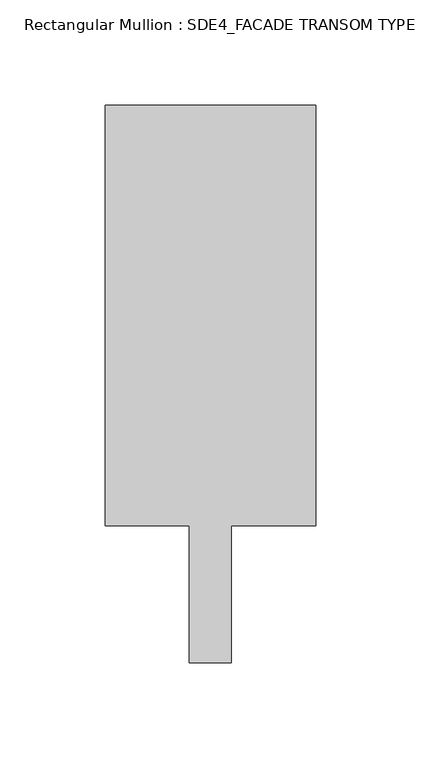
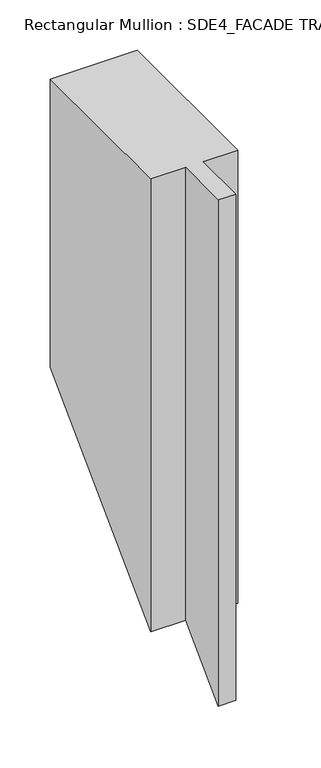
"""IFC4 building model written with IfcOpenShell, lengths in millimetres: member geometry, Rectangular Mullion : SDE4_FACADE TRANSOM TYPE 2."""

from ifc_helpers import new_model, si_unit, origin, place, context, project, spatial, faceted_brep, source, transform, mapped, element, save


def rectangular_mullion_sde4_facade_transom_type_2_aec9e63c(model_context):
    return source(origin(), model_context, "Body", "Brep", [
        faceted_brep([(50.0, 132.5, 0.0), (-50.0, 132.5, 0.0), (-50.0, -67.5, 0.0), (-10.0, -67.5, 0.0), (-10.0, -132.5, 0.0), (10.0, -132.5, 0.0), (10.0, -67.5, 0.0), (50.0, -67.5, 0.0), (50.0, 132.5, -350.4009618), (-50.0, 132.5, -350.4009618), (-50.0, -67.5, -550.4009618), (-10.0, -67.5, -550.4009618), (-10.0, -132.5, -615.4009618), (10.0, -132.5, -615.4009618), (10.0, -67.5, -550.4009618), (50.0, -67.5, -550.4009618)], [[[0, 1, 2, 3, 4, 5, 6, 7]], [[1, 0, 8, 9]], [[2, 1, 9, 10]], [[3, 2, 10, 11]], [[4, 3, 11, 12]], [[5, 4, 12, 13]], [[6, 5, 13, 14]], [[7, 6, 14, 15]], [[0, 7, 15, 8]], [[8, 15, 14, 13, 12, 11, 10, 9]]]),
    ])


if __name__ == "__main__":
    model = new_model("IFC4")
    model_context = context("Model", 3, world=origin())
    ifc_project = project(units=[si_unit("LENGTHUNIT", "METRE", prefix="MILLI")], contexts=[model_context])
    site = spatial("IfcSite", under=ifc_project)
    building = spatial("IfcBuilding", under=site)
    placement = place(None, origin())
    rectangular_mullion_sde4_facade_transom_type_2_shape = rectangular_mullion_sde4_facade_transom_type_2_aec9e63c(model_context)
    element("IfcMember", 1, ObjectType="Rectangular Mullion : SDE4_FACADE TRANSOM TYPE 2", at=placement, inside=building, context=model_context, shape_type="MappedRepresentation", body=[
        mapped(rectangular_mullion_sde4_facade_transom_type_2_shape, transform((0.0, 0.0, 0.0), x_axis=(1.0, 0.0, 0.0), y_axis=(0.0, 1.0, 0.0), z_axis=(0.0, 0.0, 1.0))),
    ])
    save(model, "model.ifc")

# Revit data of these elements
# Type "Rectangular Mullion : SDE4_FACADE TRANSOM TYPE 2"
#   built-in parameter 1007322 = 0.869423 (stored number, unit not read)
#   built-in parameter 1007321 = 0.164042 (stored number, unit not read)
#   built-in parameter 1007320 = 0.164042 (stored number, unit not read)
